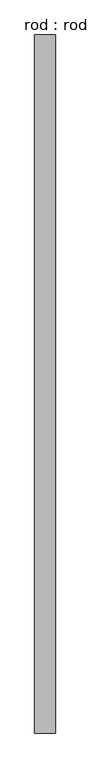
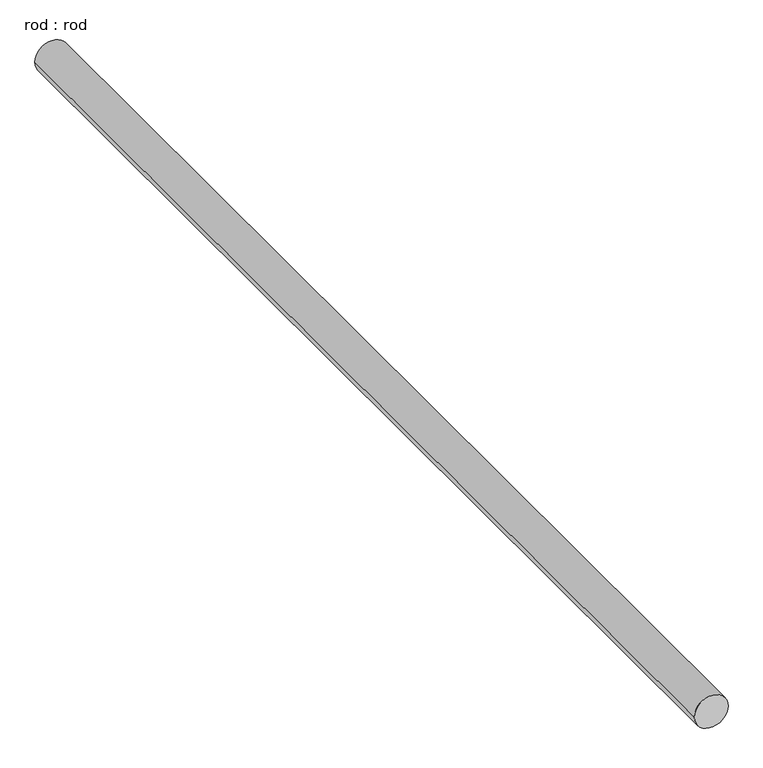
"""IFC4 building model written with IfcOpenShell, lengths in millimetres: proxy geometry, rod : rod."""

from ifc_helpers import new_model, si_unit, point, frame, frame_2d, origin, place, context, project, spatial, circle_curve, trimmed, segment, composite_curve, outline, extrude, source, transform, mapped, element, save


def rod_rod_79f9c8de(model_context):
    return source(origin(), model_context, "Body", "SweptSolid", [
        extrude(outline(composite_curve([segment(trimmed(circle_curve(frame_2d((0.0108462, 0.0)), 200.0), [point((0.0108462, 200.0))], [point((0.0108462, -200.0))], False, "CARTESIAN"), True, "CONTINUOUS"), segment(trimmed(circle_curve(frame_2d((0.0108462, 0.0)), 200.0), [point((0.0108462, -200.0))], [point((0.0108462, 200.0))], False, "CARTESIAN"), True, "CONTINUOUS")], self_intersect=False)), frame((0.0, -2664.1757182, 0.0), z_axis=(0.0, 1.0, 0.0), x_axis=(0.0, 0.0, 1.0)), (0.0, 0.0, 1.0), 13513.8086671),
    ])


if __name__ == "__main__":
    model = new_model("IFC4")
    model_context = context("Model", 3, world=origin())
    ifc_project = project(units=[si_unit("LENGTHUNIT", "METRE", prefix="MILLI")], contexts=[model_context])
    site = spatial("IfcSite", under=ifc_project)
    building = spatial("IfcBuilding", under=site)
    placement = place(None, origin())
    rod_rod_shape = rod_rod_79f9c8de(model_context)
    element("IfcBuildingElementProxy", 1, Name="rod : rod", ObjectType="rod : rod", at=placement, inside=building, context=model_context, shape_type="MappedRepresentation", body=[
        mapped(rod_rod_shape, transform((0.0, 0.0, 0.0), x_axis=(1.0, 0.0, 0.0), y_axis=(0.0, 1.0, 0.0), z_axis=(0.0, 0.0, 1.0))),
    ])
    save(model, "model.ifc")

# Revit data of these elements
# Type "rod : rod"
#   Default Elevation = 0
